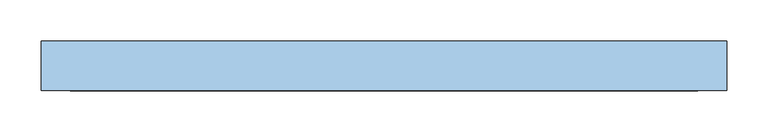
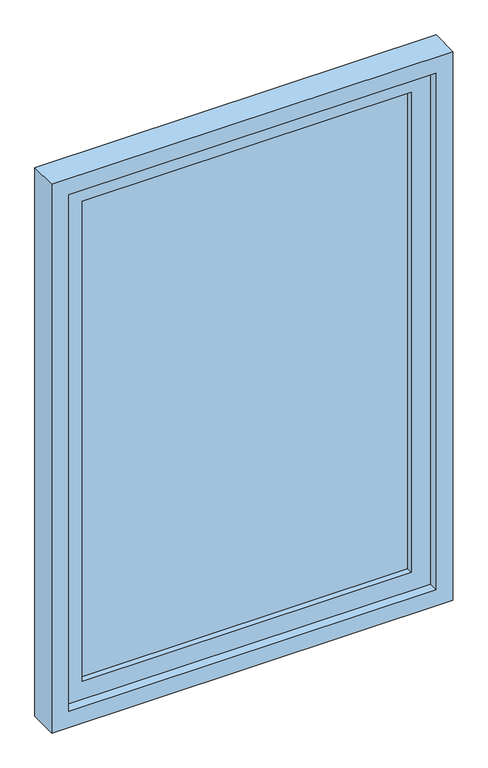
"""IFC4 building model written with IfcOpenShell, lengths in millimetres: window geometry, Janela fixa - 1 Painel : Janela fixa - 1 Painel."""

from ifc_helpers import new_model, si_unit, frame, origin, place, context, project, spatial, polyline, outline, extrude, source, transform, mapped, element, save


def window_2ae764da(model_context):
    return source(origin(), model_context, "Body", "SweptSolid", [
        extrude(outline(polyline([(340.0, 52.6), (-340.0, 52.6), (-340.0, 66.6), (340.0, 66.6), (340.0, 52.6)])), frame((0.0, 0.0, 725.0), z_axis=(0.0, 0.0, 1.0), x_axis=(1.0, 0.0, 0.0)), (0.0, 0.0, 1.0), 1050.0),
        extrude(outline(polyline([(1815.0, -380.0), (685.0, -380.0), (685.0, 380.0), (1815.0, 380.0), (1815.0, -380.0)]), holes=[polyline([(725.0, -340.0), (1775.0, -340.0), (1775.0, 340.0), (725.0, 340.0), (725.0, -340.0)])]), frame((0.0, 39.6, 0.0), z_axis=(0.0, 1.0, 0.0), x_axis=(0.0, 0.0, 1.0)), (0.0, 0.0, 1.0), 40.0),
        extrude(outline(polyline([(1850.0, -415.0), (650.0, -415.0), (650.0, 415.0), (1850.0, 415.0), (1850.0, -415.0)]), holes=[polyline([(685.0, -380.0), (1815.0, -380.0), (1815.0, 380.0), (685.0, 380.0), (685.0, -380.0)])]), frame((0.0, 19.6, 0.0), z_axis=(0.0, 1.0, 0.0), x_axis=(0.0, 0.0, 1.0)), (0.0, 0.0, 1.0), 60.0),
    ])


if __name__ == "__main__":
    model = new_model("IFC4")
    model_context = context("Model", 3, world=origin())
    ifc_project = project(units=[si_unit("LENGTHUNIT", "METRE", prefix="MILLI")], contexts=[model_context])
    site = spatial("IfcSite", under=ifc_project)
    building = spatial("IfcBuilding", under=site)
    placement = place(None, origin())
    window_shape = window_2ae764da(model_context)
    element("IfcWindow", 1, ObjectType="Janela fixa - 1 Painel : Janela fixa - 1 Painel", at=placement, inside=building, context=model_context, shape_type="MappedRepresentation", body=[
        mapped(window_shape, transform((0.0, 0.0, 0.0), x_axis=(1.0, 0.0, 0.0), y_axis=(0.0, 1.0, 0.0), z_axis=(0.0, 0.0, 1.0))),
    ])
    save(model, "model.ifc")

# Revit data of these elements
# Type "Janela fixa - 1 Painel : Janela fixa - 1 Painel"
#   Type Mark = "J15"
#   Construction Type Id = "SGL"
#   Analytic Construction = "Janelas grandes envidraçadas únicas"
#   Visual Light Transmittance = 0.9
#   Solar Heat Gain Coefficient = 0.86
#   Rough Width = 0.83 m
#   Rough Height = 1.20 m
#   Largura da moldura do painel = 0.04 m
#   Espessura da moldura do painel = 0.04 m
#   Height = 1.20 m
#   Heat Transfer Coefficient (U) = 5.5617 W/(m²·K)
#   Largura da estrutura = 0.035 m
#   Espessura da moldura = 0.06 m
#   Altura-padrão do peitoril = 0.65 m
#   Width = 0.83 m
#   Vidro = Vidro - Janela
#   Material da estrutura = Aluminum Sill
#   Wall Closure = (empty or 0)
# Element 1 (IfcWindow, "Janela fixa - 1 Painel : Janela fixa - 1 Painel")
#   Materials on its faces: "Aluminum Sill", "Vidro - Janela"
# Materials
#   "Vidro - Janela": class "Vidro", colour RGB 249 249 249, transparency 1, Cost = 0
#   "Aluminum Sill": class "Não atribuído", colour RGB 247 247 247, transparency 0
